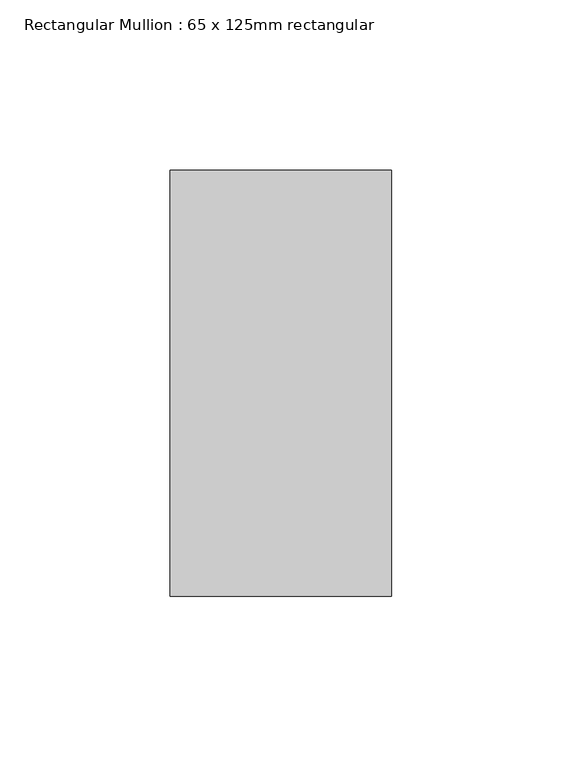
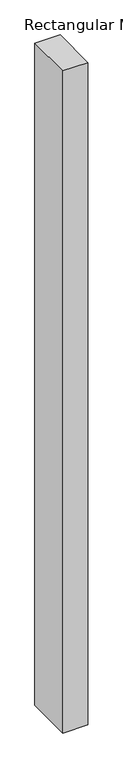
"""IFC4 building model written with IfcOpenShell, lengths in millimetres: member geometry, Rectangular Mullion : 65 x 125mm rectangular."""

from ifc_helpers import new_model, si_unit, frame, origin, place, context, project, spatial, polyline, outline, extrude, source, transform, mapped, element, save


def rectangular_mullion_65_x_125mm_rectangular_36adfa9f(model_context):
    return source(origin(), model_context, "Body", "SweptSolid", [
        extrude(outline(polyline([(0.0, 62.5), (0.0, -62.5), (-65.0, -62.5), (-65.0, 62.5), (0.0, 62.5)])), frame((0.0, 0.0, -1809.1666668), z_axis=(0.0, 0.0, 1.0), x_axis=(1.0, 0.0, 0.0)), (0.0, 0.0, 1.0), 1809.1666668),
    ])


if __name__ == "__main__":
    model = new_model("IFC4")
    model_context = context("Model", 3, world=origin())
    ifc_project = project(units=[si_unit("LENGTHUNIT", "METRE", prefix="MILLI")], contexts=[model_context])
    site = spatial("IfcSite", under=ifc_project)
    building = spatial("IfcBuilding", under=site)
    placement = place(None, origin())
    rectangular_mullion_65_x_125mm_rectangular_shape = rectangular_mullion_65_x_125mm_rectangular_36adfa9f(model_context)
    element("IfcMember", 1, ObjectType="Rectangular Mullion : 65 x 125mm rectangular", at=placement, inside=building, context=model_context, shape_type="MappedRepresentation", body=[
        mapped(rectangular_mullion_65_x_125mm_rectangular_shape, transform((0.0, 0.0, 0.0), x_axis=(1.0, 0.0, 0.0), y_axis=(0.0, 1.0, 0.0), z_axis=(0.0, 0.0, 1.0))),
    ])
    save(model, "model.ifc")

# Revit data of these elements
# Type "Rectangular Mullion : 65 x 125mm rectangular"
#   built-in parameter 1007304 = 0.410105 (stored number, unit not read)
#   built-in parameter 1007301 = 0.106627 (stored number, unit not read)
#   built-in parameter 1007300 = 0.106627 (stored number, unit not read)
# Element 1 (IfcMember, "Rectangular Mullion : 65 x 125mm rectangular")
#   Materials on its faces: "Aluminum"
# Materials
#   "Aluminum": class "Metal", colour RGB 244 245 246, transparency 0, Description = "Aluminum 6061", Cost = 0
